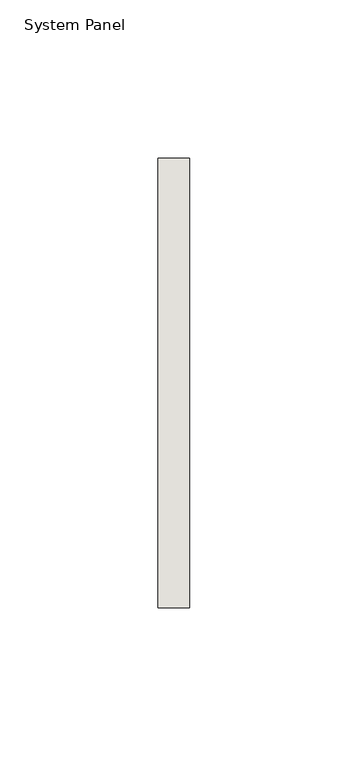
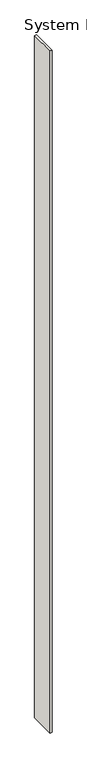
"""IFC4 building model written with IfcOpenShell, lengths in millimetres: wall geometry, System Panel : NLRS_21_CWP_hsb-vulling minerale wol 142 _gen_rsf."""

import ifcopenshell
import ifcopenshell.guid

model = None  # the IFC model being written
_history = None  # IfcOwnerHistory: only IFC2X3 demands one
_inside = {}  # id of a spatial element -> (the spatial element, [elements in it])
_under = {}  # id of a project, library or spatial element -> (it, [spatial elements below it])
_declared = {}  # id of a project -> (the project, [libraries it declares])
_typed = {}  # id of a type object -> (the type object, [elements of that type])
_made_of = {}  # id of a material, layer set ... -> (it, [elements and type objects made of it])


def new_model(schema):
    """Start an empty IFC model of exactly this schema.

    Asked for "IFC4X3", IfcOpenShell would pick the latest addendum, in which some entities
    have other attributes; the version numbers below select the first issue.
    IFC2X3 requires an IfcOwnerHistory on every rooted entity: one is made here for all.
    """
    global model, _history
    if schema == "IFC4X3":
        model = ifcopenshell.file(schema_version=(4, 3, 0, 0))
    else:
        model = ifcopenshell.file(schema=schema)
    _inside.clear()
    _under.clear()
    _declared.clear()
    _typed.clear()
    _made_of.clear()
    _history = None
    if model.schema == "IFC2X3":
        org = make("IfcOrganization", Name="unknown")
        user = make(
            "IfcPersonAndOrganization",
            ThePerson=make("IfcPerson", FamilyName="unknown"),
            TheOrganization=org,
        )
        app = make(
            "IfcApplication",
            ApplicationDeveloper=org,
            Version="unknown",
            ApplicationFullName="unknown",
            ApplicationIdentifier="unknown",
        )
        _history = make(
            "IfcOwnerHistory",
            OwningUser=user,
            OwningApplication=app,
            ChangeAction="ADDED",
            CreationDate=0,
        )
    return model


def make(cls, **values):
    """One entity of the class cls with the attributes given. An attribute that is None is left unset."""
    return model.create_entity(
        cls, **{name: value for name, value in values.items() if value is not None}
    )


def rooted(cls, **values):
    """An entity with a GlobalId (a new one), such as an element, a storey or a relation."""
    return make(cls, GlobalId=ifcopenshell.guid.new(), OwnerHistory=_history, **values)


def si_unit(unit_type, name, prefix=None):
    """IfcSIUnit, for example si_unit("LENGTHUNIT", "METRE", prefix="MILLI")."""
    return make("IfcSIUnit", UnitType=unit_type, Prefix=prefix, Name=name)


def assignment(units):
    """IfcUnitAssignment: the units of a project."""
    return None if units is None else make("IfcUnitAssignment", Units=units)


def point(xyz):
    """IfcCartesianPoint."""
    return None if xyz is None else make("IfcCartesianPoint", Coordinates=xyz)


def direction(xyz):
    """IfcDirection."""
    return None if xyz is None else make("IfcDirection", DirectionRatios=xyz)


def frame(location, z_axis=None, x_axis=None):
    """IfcAxis2Placement3D, a coordinate frame: its origin and axes. An axis left out is left unset."""
    return make(
        "IfcAxis2Placement3D",
        Location=point(location),
        Axis=direction(z_axis),
        RefDirection=direction(x_axis),
    )


def origin():
    """The frame at (0, 0, 0) with its axes left unset."""
    return frame((0.0, 0.0, 0.0))


def origin_with_axes():
    """The frame at (0, 0, 0) with the z axis (0, 0, 1) and the x axis (1, 0, 0) written out."""
    return frame((0.0, 0.0, 0.0), z_axis=(0.0, 0.0, 1.0), x_axis=(1.0, 0.0, 0.0))


def place(relative_to, where):
    """IfcLocalPlacement: puts the frame where relative to a parent placement (None: the world)."""
    return make(
        "IfcLocalPlacement", PlacementRelTo=relative_to, RelativePlacement=where
    )


def context(
    kind, dimensions, precision=None, world=None, true_north=None, identifier=None
):
    """IfcGeometricRepresentationContext, for example the 3D "Model" context."""
    return make(
        "IfcGeometricRepresentationContext",
        ContextIdentifier=identifier,
        ContextType=kind,
        CoordinateSpaceDimension=dimensions,
        Precision=precision,
        WorldCoordinateSystem=world,
        TrueNorth=true_north,
    )


def project(units=None, contexts=None):
    """IfcProject with its units and contexts."""
    return rooted(
        "IfcProject",
        Name="project",
        RepresentationContexts=contexts,
        UnitsInContext=assignment(units),
    )


def spatial(cls, under=None, at=None, **own):
    """A site, building, storey or space (cls), placed at a placement, below another one or the project."""
    s = rooted(cls, ObjectPlacement=at, **own)
    if under is not None:
        _under.setdefault(under.id(), (under, []))[1].append(s)
    return s


def polyline(points):
    """IfcPolyline through the points."""
    return make("IfcPolyline", Points=[point(p) for p in points])


def outline(outer, holes=None, kind="AREA"):
    """IfcArbitraryClosedProfileDef: a profile drawn as a closed curve; with holes, ...WithVoids."""
    if holes is None:
        return make("IfcArbitraryClosedProfileDef", ProfileType=kind, OuterCurve=outer)
    return make(
        "IfcArbitraryProfileDefWithVoids",
        ProfileType=kind,
        OuterCurve=outer,
        InnerCurves=holes,
    )


def extrude(swept, where, along, depth):
    """IfcExtrudedAreaSolid: the profile swept, set in the frame where, extruded along a direction by depth."""
    return make(
        "IfcExtrudedAreaSolid",
        SweptArea=swept,
        Position=where,
        ExtrudedDirection=direction(along),
        Depth=depth,
    )


def shape(context_of_items, identifier, shape_type, items):
    """IfcShapeRepresentation: the items that make up one representation, for example the "Body"."""
    return make(
        "IfcShapeRepresentation",
        ContextOfItems=context_of_items,
        RepresentationIdentifier=identifier,
        RepresentationType=shape_type,
        Items=items,
    )


def source(mapping_origin, context_of_items, identifier, shape_type, items):
    """IfcRepresentationMap: a shape defined once, which mapped items show again and again."""
    return make(
        "IfcRepresentationMap",
        MappingOrigin=mapping_origin,
        MappedRepresentation=shape(context_of_items, identifier, shape_type, items),
    )


def transform(
    local_origin,
    x_axis=None,
    y_axis=None,
    z_axis=None,
    scale=None,
    scale2=None,
    scale3=None,
    uniform=True,
):
    """IfcCartesianTransformationOperator3D, or its non-uniform kind. x_axis, y_axis, z_axis: its Axis1, 2, 3."""
    if uniform:
        return make(
            "IfcCartesianTransformationOperator3D",
            Axis1=direction(x_axis),
            Axis2=direction(y_axis),
            LocalOrigin=point(local_origin),
            Scale=scale,
            Axis3=direction(z_axis),
        )
    return make(
        "IfcCartesianTransformationOperator3DnonUniform",
        Axis1=direction(x_axis),
        Axis2=direction(y_axis),
        LocalOrigin=point(local_origin),
        Scale=scale,
        Axis3=direction(z_axis),
        Scale2=scale2,
        Scale3=scale3,
    )


def mapped(mapping_source, mapping_target):
    """IfcMappedItem: shows the shape of a source again, moved by a transform."""
    return make(
        "IfcMappedItem", MappingSource=mapping_source, MappingTarget=mapping_target
    )


def made_of(thing, what):
    """Note that an element or type object is made of a material, layer set ...; save() writes the relation."""
    if what is not None:
        _made_of.setdefault(what.id(), (what, []))[1].append(thing)
    return thing


def element(
    cls,
    number,
    at=None,
    inside=None,
    cuts=None,
    type_object=None,
    material=None,
    context=None,
    identifier="Body",
    shape_type=None,
    held_by="IfcProductDefinitionShape",
    body=None,
    shapes=None,
    **own,
):
    """One element of the class cls, such as IfcWall. Its Tag is "e" and its number.

    at: its placement. inside: the storey or other place that contains it. cuts: it is an
    opening in that element (IfcRelVoidsElement). A single representation is given by context,
    identifier, shape_type and body (its items); several are given by shapes. held_by: the class
    of the entity that holds the representations. save() writes the other relations.
    """
    e = rooted(cls, Tag="e%d" % number, ObjectPlacement=at, **own)
    if body is not None:
        shapes = [shape(context, identifier, shape_type, body)]
    if shapes is not None:
        e.Representation = make(held_by, Representations=shapes)
    if inside is not None:
        _inside.setdefault(inside.id(), (inside, []))[1].append(e)
    if cuts is not None:
        rooted(
            "IfcRelVoidsElement", RelatingBuildingElement=cuts, RelatedOpeningElement=e
        )
    if type_object is not None:
        _typed.setdefault(type_object.id(), (type_object, []))[1].append(e)
    return made_of(e, material)


def aggregate(whole, parts):
    """IfcRelAggregates: a whole, such as a stair, and the parts it consists of."""
    return rooted("IfcRelAggregates", RelatingObject=whole, RelatedObjects=parts)


def save(model, path):
    """Write the relations noted so far, then the file.

    IfcRelAggregates (storeys below a building ...), IfcRelContainedInSpatialStructure (elements
    in a storey), IfcRelDefinesByType, IfcRelAssociatesMaterial and IfcRelDeclares: one each for
    every whole, place, type object, material and project.
    """
    for whole, parts in _under.values():
        aggregate(whole, parts)
    for where, things in _inside.values():
        rooted(
            "IfcRelContainedInSpatialStructure",
            RelatedElements=things,
            RelatingStructure=where,
        )
    for kind, things in _typed.values():
        rooted("IfcRelDefinesByType", RelatedObjects=things, RelatingType=kind)
    for what, things in _made_of.values():
        rooted("IfcRelAssociatesMaterial", RelatedObjects=things, RelatingMaterial=what)
    for by, libraries in _declared.values():
        rooted("IfcRelDeclares", RelatingContext=by, RelatedDefinitions=libraries)
    model.write(path)


def system_panel_1da55d1c(model_context):
    return source(origin(), model_context, "Body", "SweptSolid", [
        extrude(outline(polyline([(4.9999998, -71.0), (-4.9999998, -71.0), (-4.9999998, 71.0), (4.9999998, 71.0), (4.9999998, -71.0)])), origin_with_axes(), (0.0, 0.0, 1.0), 3849.0),
    ])


if __name__ == "__main__":
    model = new_model("IFC4")
    model_context = context("Model", 3, world=origin())
    ifc_project = project(units=[si_unit("LENGTHUNIT", "METRE", prefix="MILLI")], contexts=[model_context])
    site = spatial("IfcSite", under=ifc_project)
    building = spatial("IfcBuilding", under=site)
    placement = place(None, origin())
    system_panel_shape = system_panel_1da55d1c(model_context)
    element("IfcWall", 1, ObjectType="System Panel : NLRS_21_CWP_hsb-vulling minerale wol 142 _gen_rsf", at=placement, inside=building, context=model_context, shape_type="MappedRepresentation", body=[
        mapped(system_panel_shape, transform((0.0, 0.0, 0.0), x_axis=(1.0, 0.0, 0.0), y_axis=(0.0, 1.0, 0.0), z_axis=(0.0, 0.0, 1.0))),
    ])
    save(model, "model.ifc")

# Revit data of these elements
# Type "System Panel : NLRS_21_CWP_hsb-vulling minerale wol 142 _gen_rsf"
#   Type IfcGUID = "07M7mRoiH1CR8m_RSKIwpC"
#   Assembly Code = "21.23"
#   IfcExportAs = "IfcWall"
# Element 1 (IfcWall, "System Panel : NLRS_21_CWP_hsb-vulling minerale wol 142 _gen_rsf")
#   Materials on its faces: "NLRS_m1_isolatie minerale wol_gen_rsf"
# Materials
#   "NLRS_m1_isolatie minerale wol_gen_rsf": class "M - Anorganische materialen", colour RGB 200 200 140, transparency 0, Keynote = "m1", Manufacturer = "Revit Standards Foundation", URL = "www.revitstandards.org", Description = "isolatie minerale wol", Cost = 0
